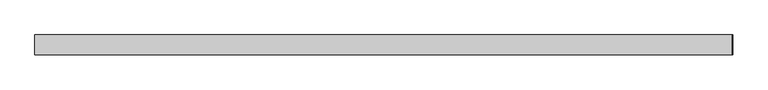
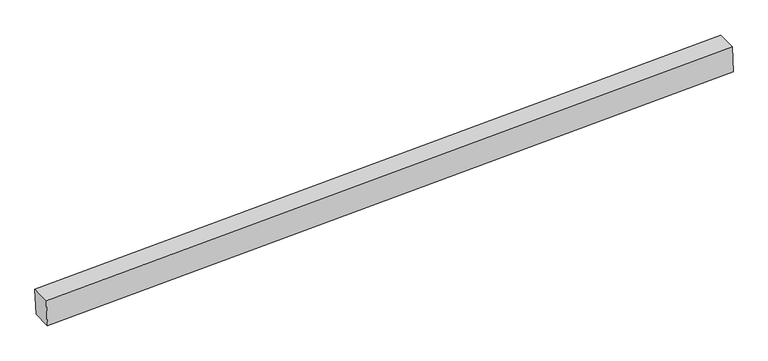
"""IFC4 building model written with IfcOpenShell, lengths in millimetres: proxy geometry, Generic Models 7:Generic Models 1:8:Generic Models 1:8 : Generic Models 7:Generic Models 1:337419:30 : Generic Models 7:Generic Models 1:8:Generic Models 1:8 : Generic Models 7:Generic Models 1:337419:315935."""

from ifc_helpers import new_model, si_unit, frame, origin, place, context, project, spatial, polyline, outline, extrude, source, transform, mapped, element, save


def generic_models_890d81a9(model_context):
    return source(origin(), model_context, "Body", "SweptSolid", [
        extrude(outline(polyline([(3818.9012888, 558136.9256261), (3628.5664384, 558144.8562449), (3831.5897382, 563017.4154421), (4021.9397427, 563009.8485204), (3818.9012888, 558136.9256261)])), frame((0.0, -577565.5913841, 0.0), z_axis=(0.0, 1.0, 0.0), x_axis=(0.0, 0.0, 1.0)), (0.0, 0.0, 1.0), 139.7),
    ])


if __name__ == "__main__":
    model = new_model("IFC4")
    model_context = context("Model", 3, world=origin())
    ifc_project = project(units=[si_unit("LENGTHUNIT", "METRE", prefix="MILLI")], contexts=[model_context])
    site = spatial("IfcSite", under=ifc_project)
    building = spatial("IfcBuilding", under=site)
    placement = place(None, origin())
    generic_models_shape = generic_models_890d81a9(model_context)
    element("IfcBuildingElementProxy", 1, Name="Generic Models 7:Generic Models 1:8:Generic Models 1:8 : Generic Models 7:Generic Models 1:337419:30 : Generic Models 7:Generic Models 1:8:Generic Models 1:8 : Generic Models 7:Generic Models 1:337419:315935", ObjectType="Generic Models 7:Generic Models 1:8:Generic Models 1:8 : Generic Models 7:Generic Models 1:337419:30 : Generic Models 7:Generic Models 1:8:Generic Models 1:8 : Generic Models 7:Generic Models 1:337419:315935", at=placement, inside=building, context=model_context, shape_type="MappedRepresentation", body=[
        mapped(generic_models_shape, transform((0.0, 0.0, 0.0), x_axis=(1.0, 0.0, 0.0), y_axis=(0.0, 1.0, 0.0), z_axis=(0.0, 0.0, 1.0))),
    ])
    save(model, "model.ifc")

# Revit data of these elements
# Type "Generic Models 7:Generic Models 1:8:Generic Models 1:8 : Generic Models 7:Generic Models 1:337419:30 : Generic Models 7:Generic Models 1:8:Generic Models 1:8 : Generic Models 7:Generic Models 1:337419:315935"
#   NameOverride = "Generic Models 7:Generic Models 1:8:Generic Models 1:8 : Generic Models 7:Generic Models 1:337419:315935"
#   ObjectTypeOverride = "Generic Models 1:8 : Generic Models 7:Generic Models 1:337419"
#   Reference = "Generic Models 1"
#   Tag = "315935"
# Element 1 (IfcBuildingElementProxy, "Generic Models 7:Generic Models 1:8:Generic Models 1:8 : Generic Models 7:Generic Models 1:337419:30 : Generic Models 7:Generic Models 1:8:Generic Models 1:8 : Generic Models 7:Generic Models 1:337419:315935")
#   Materials on its faces: "5 1/8\" X 7 1/2\" EXTERIOR GRADE GLULAM BEAMS (4'- 0 1/4\" O.C.)"
# Materials
#   "5 1/8\" X 7 1/2\" EXTERIOR GRADE GLULAM BEAMS (4'- 0 1/4\" O.C.)": class "Wood", colour RGB 183 134 68, transparency 0, Keynote = "M06181300.01", Description = "Pinus Echinata", Cost = 0
